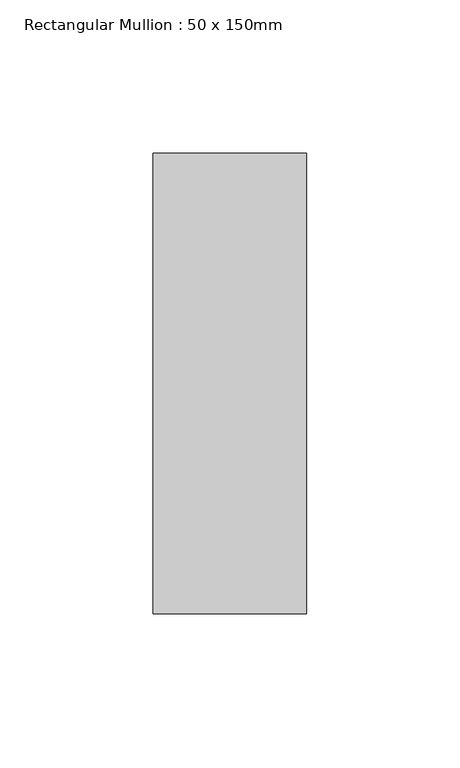
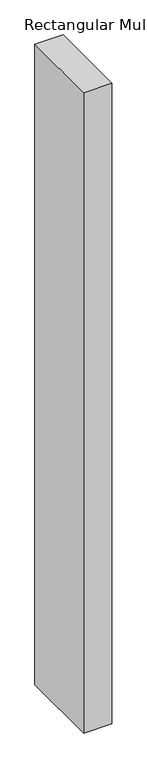
"""IFC4 building model written with IfcOpenShell, lengths in millimetres: member geometry, Rectangular Mullion : 50 x 150mm."""

import ifcopenshell
import ifcopenshell.guid

model = None  # the IFC model being written
_history = None  # IfcOwnerHistory: only IFC2X3 demands one
_inside = {}  # id of a spatial element -> (the spatial element, [elements in it])
_under = {}  # id of a project, library or spatial element -> (it, [spatial elements below it])
_declared = {}  # id of a project -> (the project, [libraries it declares])
_typed = {}  # id of a type object -> (the type object, [elements of that type])
_made_of = {}  # id of a material, layer set ... -> (it, [elements and type objects made of it])


def new_model(schema):
    """Start an empty IFC model of exactly this schema.

    Asked for "IFC4X3", IfcOpenShell would pick the latest addendum, in which some entities
    have other attributes; the version numbers below select the first issue.
    IFC2X3 requires an IfcOwnerHistory on every rooted entity: one is made here for all.
    """
    global model, _history
    if schema == "IFC4X3":
        model = ifcopenshell.file(schema_version=(4, 3, 0, 0))
    else:
        model = ifcopenshell.file(schema=schema)
    _inside.clear()
    _under.clear()
    _declared.clear()
    _typed.clear()
    _made_of.clear()
    _history = None
    if model.schema == "IFC2X3":
        org = make("IfcOrganization", Name="unknown")
        user = make(
            "IfcPersonAndOrganization",
            ThePerson=make("IfcPerson", FamilyName="unknown"),
            TheOrganization=org,
        )
        app = make(
            "IfcApplication",
            ApplicationDeveloper=org,
            Version="unknown",
            ApplicationFullName="unknown",
            ApplicationIdentifier="unknown",
        )
        _history = make(
            "IfcOwnerHistory",
            OwningUser=user,
            OwningApplication=app,
            ChangeAction="ADDED",
            CreationDate=0,
        )
    return model


def make(cls, **values):
    """One entity of the class cls with the attributes given. An attribute that is None is left unset."""
    return model.create_entity(
        cls, **{name: value for name, value in values.items() if value is not None}
    )


def rooted(cls, **values):
    """An entity with a GlobalId (a new one), such as an element, a storey or a relation."""
    return make(cls, GlobalId=ifcopenshell.guid.new(), OwnerHistory=_history, **values)


def si_unit(unit_type, name, prefix=None):
    """IfcSIUnit, for example si_unit("LENGTHUNIT", "METRE", prefix="MILLI")."""
    return make("IfcSIUnit", UnitType=unit_type, Prefix=prefix, Name=name)


def assignment(units):
    """IfcUnitAssignment: the units of a project."""
    return None if units is None else make("IfcUnitAssignment", Units=units)


def point(xyz):
    """IfcCartesianPoint."""
    return None if xyz is None else make("IfcCartesianPoint", Coordinates=xyz)


def direction(xyz):
    """IfcDirection."""
    return None if xyz is None else make("IfcDirection", DirectionRatios=xyz)


def frame(location, z_axis=None, x_axis=None):
    """IfcAxis2Placement3D, a coordinate frame: its origin and axes. An axis left out is left unset."""
    return make(
        "IfcAxis2Placement3D",
        Location=point(location),
        Axis=direction(z_axis),
        RefDirection=direction(x_axis),
    )


def origin():
    """The frame at (0, 0, 0) with its axes left unset."""
    return frame((0.0, 0.0, 0.0))


def place(relative_to, where):
    """IfcLocalPlacement: puts the frame where relative to a parent placement (None: the world)."""
    return make(
        "IfcLocalPlacement", PlacementRelTo=relative_to, RelativePlacement=where
    )


def context(
    kind, dimensions, precision=None, world=None, true_north=None, identifier=None
):
    """IfcGeometricRepresentationContext, for example the 3D "Model" context."""
    return make(
        "IfcGeometricRepresentationContext",
        ContextIdentifier=identifier,
        ContextType=kind,
        CoordinateSpaceDimension=dimensions,
        Precision=precision,
        WorldCoordinateSystem=world,
        TrueNorth=true_north,
    )


def project(units=None, contexts=None):
    """IfcProject with its units and contexts."""
    return rooted(
        "IfcProject",
        Name="project",
        RepresentationContexts=contexts,
        UnitsInContext=assignment(units),
    )


def spatial(cls, under=None, at=None, **own):
    """A site, building, storey or space (cls), placed at a placement, below another one or the project."""
    s = rooted(cls, ObjectPlacement=at, **own)
    if under is not None:
        _under.setdefault(under.id(), (under, []))[1].append(s)
    return s


def polyline(points):
    """IfcPolyline through the points."""
    return make("IfcPolyline", Points=[point(p) for p in points])


def outline(outer, holes=None, kind="AREA"):
    """IfcArbitraryClosedProfileDef: a profile drawn as a closed curve; with holes, ...WithVoids."""
    if holes is None:
        return make("IfcArbitraryClosedProfileDef", ProfileType=kind, OuterCurve=outer)
    return make(
        "IfcArbitraryProfileDefWithVoids",
        ProfileType=kind,
        OuterCurve=outer,
        InnerCurves=holes,
    )


def extrude(swept, where, along, depth):
    """IfcExtrudedAreaSolid: the profile swept, set in the frame where, extruded along a direction by depth."""
    return make(
        "IfcExtrudedAreaSolid",
        SweptArea=swept,
        Position=where,
        ExtrudedDirection=direction(along),
        Depth=depth,
    )


def shape(context_of_items, identifier, shape_type, items):
    """IfcShapeRepresentation: the items that make up one representation, for example the "Body"."""
    return make(
        "IfcShapeRepresentation",
        ContextOfItems=context_of_items,
        RepresentationIdentifier=identifier,
        RepresentationType=shape_type,
        Items=items,
    )


def source(mapping_origin, context_of_items, identifier, shape_type, items):
    """IfcRepresentationMap: a shape defined once, which mapped items show again and again."""
    return make(
        "IfcRepresentationMap",
        MappingOrigin=mapping_origin,
        MappedRepresentation=shape(context_of_items, identifier, shape_type, items),
    )


def transform(
    local_origin,
    x_axis=None,
    y_axis=None,
    z_axis=None,
    scale=None,
    scale2=None,
    scale3=None,
    uniform=True,
):
    """IfcCartesianTransformationOperator3D, or its non-uniform kind. x_axis, y_axis, z_axis: its Axis1, 2, 3."""
    if uniform:
        return make(
            "IfcCartesianTransformationOperator3D",
            Axis1=direction(x_axis),
            Axis2=direction(y_axis),
            LocalOrigin=point(local_origin),
            Scale=scale,
            Axis3=direction(z_axis),
        )
    return make(
        "IfcCartesianTransformationOperator3DnonUniform",
        Axis1=direction(x_axis),
        Axis2=direction(y_axis),
        LocalOrigin=point(local_origin),
        Scale=scale,
        Axis3=direction(z_axis),
        Scale2=scale2,
        Scale3=scale3,
    )


def mapped(mapping_source, mapping_target):
    """IfcMappedItem: shows the shape of a source again, moved by a transform."""
    return make(
        "IfcMappedItem", MappingSource=mapping_source, MappingTarget=mapping_target
    )


def made_of(thing, what):
    """Note that an element or type object is made of a material, layer set ...; save() writes the relation."""
    if what is not None:
        _made_of.setdefault(what.id(), (what, []))[1].append(thing)
    return thing


def element(
    cls,
    number,
    at=None,
    inside=None,
    cuts=None,
    type_object=None,
    material=None,
    context=None,
    identifier="Body",
    shape_type=None,
    held_by="IfcProductDefinitionShape",
    body=None,
    shapes=None,
    **own,
):
    """One element of the class cls, such as IfcWall. Its Tag is "e" and its number.

    at: its placement. inside: the storey or other place that contains it. cuts: it is an
    opening in that element (IfcRelVoidsElement). A single representation is given by context,
    identifier, shape_type and body (its items); several are given by shapes. held_by: the class
    of the entity that holds the representations. save() writes the other relations.
    """
    e = rooted(cls, Tag="e%d" % number, ObjectPlacement=at, **own)
    if body is not None:
        shapes = [shape(context, identifier, shape_type, body)]
    if shapes is not None:
        e.Representation = make(held_by, Representations=shapes)
    if inside is not None:
        _inside.setdefault(inside.id(), (inside, []))[1].append(e)
    if cuts is not None:
        rooted(
            "IfcRelVoidsElement", RelatingBuildingElement=cuts, RelatedOpeningElement=e
        )
    if type_object is not None:
        _typed.setdefault(type_object.id(), (type_object, []))[1].append(e)
    return made_of(e, material)


def aggregate(whole, parts):
    """IfcRelAggregates: a whole, such as a stair, and the parts it consists of."""
    return rooted("IfcRelAggregates", RelatingObject=whole, RelatedObjects=parts)


def save(model, path):
    """Write the relations noted so far, then the file.

    IfcRelAggregates (storeys below a building ...), IfcRelContainedInSpatialStructure (elements
    in a storey), IfcRelDefinesByType, IfcRelAssociatesMaterial and IfcRelDeclares: one each for
    every whole, place, type object, material and project.
    """
    for whole, parts in _under.values():
        aggregate(whole, parts)
    for where, things in _inside.values():
        rooted(
            "IfcRelContainedInSpatialStructure",
            RelatedElements=things,
            RelatingStructure=where,
        )
    for kind, things in _typed.values():
        rooted("IfcRelDefinesByType", RelatedObjects=things, RelatingType=kind)
    for what, things in _made_of.values():
        rooted("IfcRelAssociatesMaterial", RelatedObjects=things, RelatingMaterial=what)
    for by, libraries in _declared.values():
        rooted("IfcRelDeclares", RelatingContext=by, RelatedDefinitions=libraries)
    model.write(path)


def rectangular_mullion_50_x_150mm_6588f46c(model_context):
    return source(origin(), model_context, "Body", "SweptSolid", [
        extrude(outline(polyline([(0.0, 75.0), (0.0, -75.0), (-50.0, -75.0), (-50.0, 75.0), (0.0, 75.0)])), frame((0.0, 0.0, -1200.0), z_axis=(0.0, 0.0, 1.0), x_axis=(1.0, 0.0, 0.0)), (0.0, 0.0, 1.0), 1200.0),
    ])


if __name__ == "__main__":
    model = new_model("IFC4")
    model_context = context("Model", 3, world=origin())
    ifc_project = project(units=[si_unit("LENGTHUNIT", "METRE", prefix="MILLI")], contexts=[model_context])
    site = spatial("IfcSite", under=ifc_project)
    building = spatial("IfcBuilding", under=site)
    placement = place(None, origin())
    rectangular_mullion_50_x_150mm_shape = rectangular_mullion_50_x_150mm_6588f46c(model_context)
    element("IfcMember", 1, ObjectType="Rectangular Mullion : 50 x 150mm", at=placement, inside=building, context=model_context, shape_type="MappedRepresentation", body=[
        mapped(rectangular_mullion_50_x_150mm_shape, transform((0.0, 0.0, 0.0), x_axis=(1.0, 0.0, 0.0), y_axis=(0.0, 1.0, 0.0), z_axis=(0.0, 0.0, 1.0))),
    ])
    save(model, "model.ifc")

# Revit data of these elements
# Type "Rectangular Mullion : 50 x 150mm"
#   built-in parameter 1007304 = 0.492126 (stored number, unit not read)
#   built-in parameter 1007301 = 0.082021 (stored number, unit not read)
#   built-in parameter 1007300 = 0.082021 (stored number, unit not read)
# Element 1 (IfcMember, "Rectangular Mullion : 50 x 150mm")
#   Materials on its faces: "Aluminium"
# Materials
#   "Aluminium": class "Metal", colour RGB 247 247 247, transparency 0, Description = "Aluminium 6061", Cost = 0
